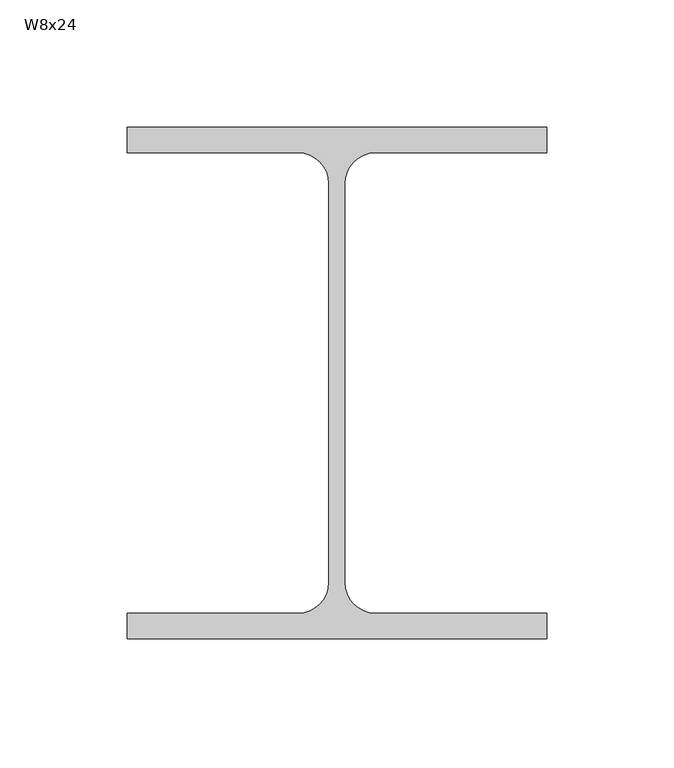
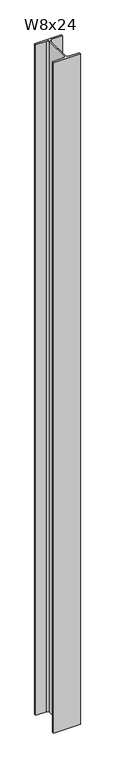
"""IFC4 building model written with IfcOpenShell, lengths in millimetres: column geometry, RME WF - Column : W8x24."""

import ifcopenshell
import ifcopenshell.guid

model = None  # the IFC model being written
_history = None  # IfcOwnerHistory: only IFC2X3 demands one
_inside = {}  # id of a spatial element -> (the spatial element, [elements in it])
_under = {}  # id of a project, library or spatial element -> (it, [spatial elements below it])
_declared = {}  # id of a project -> (the project, [libraries it declares])
_typed = {}  # id of a type object -> (the type object, [elements of that type])
_made_of = {}  # id of a material, layer set ... -> (it, [elements and type objects made of it])


def new_model(schema):
    """Start an empty IFC model of exactly this schema.

    Asked for "IFC4X3", IfcOpenShell would pick the latest addendum, in which some entities
    have other attributes; the version numbers below select the first issue.
    IFC2X3 requires an IfcOwnerHistory on every rooted entity: one is made here for all.
    """
    global model, _history
    if schema == "IFC4X3":
        model = ifcopenshell.file(schema_version=(4, 3, 0, 0))
    else:
        model = ifcopenshell.file(schema=schema)
    _inside.clear()
    _under.clear()
    _declared.clear()
    _typed.clear()
    _made_of.clear()
    _history = None
    if model.schema == "IFC2X3":
        org = make("IfcOrganization", Name="unknown")
        user = make(
            "IfcPersonAndOrganization",
            ThePerson=make("IfcPerson", FamilyName="unknown"),
            TheOrganization=org,
        )
        app = make(
            "IfcApplication",
            ApplicationDeveloper=org,
            Version="unknown",
            ApplicationFullName="unknown",
            ApplicationIdentifier="unknown",
        )
        _history = make(
            "IfcOwnerHistory",
            OwningUser=user,
            OwningApplication=app,
            ChangeAction="ADDED",
            CreationDate=0,
        )
    return model


def make(cls, **values):
    """One entity of the class cls with the attributes given. An attribute that is None is left unset."""
    return model.create_entity(
        cls, **{name: value for name, value in values.items() if value is not None}
    )


def rooted(cls, **values):
    """An entity with a GlobalId (a new one), such as an element, a storey or a relation."""
    return make(cls, GlobalId=ifcopenshell.guid.new(), OwnerHistory=_history, **values)


def si_unit(unit_type, name, prefix=None):
    """IfcSIUnit, for example si_unit("LENGTHUNIT", "METRE", prefix="MILLI")."""
    return make("IfcSIUnit", UnitType=unit_type, Prefix=prefix, Name=name)


def assignment(units):
    """IfcUnitAssignment: the units of a project."""
    return None if units is None else make("IfcUnitAssignment", Units=units)


def point(xyz):
    """IfcCartesianPoint."""
    return None if xyz is None else make("IfcCartesianPoint", Coordinates=xyz)


def direction(xyz):
    """IfcDirection."""
    return None if xyz is None else make("IfcDirection", DirectionRatios=xyz)


def frame(location, z_axis=None, x_axis=None):
    """IfcAxis2Placement3D, a coordinate frame: its origin and axes. An axis left out is left unset."""
    return make(
        "IfcAxis2Placement3D",
        Location=point(location),
        Axis=direction(z_axis),
        RefDirection=direction(x_axis),
    )


def frame_2d(location, x_axis=None):
    """IfcAxis2Placement2D, a coordinate frame in the plane: its origin and x axis."""
    return make(
        "IfcAxis2Placement2D", Location=point(location), RefDirection=direction(x_axis)
    )


def origin():
    """The frame at (0, 0, 0) with its axes left unset."""
    return frame((0.0, 0.0, 0.0))


def place(relative_to, where):
    """IfcLocalPlacement: puts the frame where relative to a parent placement (None: the world)."""
    return make(
        "IfcLocalPlacement", PlacementRelTo=relative_to, RelativePlacement=where
    )


def context(
    kind, dimensions, precision=None, world=None, true_north=None, identifier=None
):
    """IfcGeometricRepresentationContext, for example the 3D "Model" context."""
    return make(
        "IfcGeometricRepresentationContext",
        ContextIdentifier=identifier,
        ContextType=kind,
        CoordinateSpaceDimension=dimensions,
        Precision=precision,
        WorldCoordinateSystem=world,
        TrueNorth=true_north,
    )


def project(units=None, contexts=None):
    """IfcProject with its units and contexts."""
    return rooted(
        "IfcProject",
        Name="project",
        RepresentationContexts=contexts,
        UnitsInContext=assignment(units),
    )


def spatial(cls, under=None, at=None, **own):
    """A site, building, storey or space (cls), placed at a placement, below another one or the project."""
    s = rooted(cls, ObjectPlacement=at, **own)
    if under is not None:
        _under.setdefault(under.id(), (under, []))[1].append(s)
    return s


def polyline(points):
    """IfcPolyline through the points."""
    return make("IfcPolyline", Points=[point(p) for p in points])


def circle_curve(where, radius):
    """IfcCircle in the frame where."""
    return make("IfcCircle", Position=where, Radius=radius)


def trimmed(basis, trim1, trim2, sense, master):
    """IfcTrimmedCurve: the piece of a basis curve between two trims."""
    return make(
        "IfcTrimmedCurve",
        BasisCurve=basis,
        Trim1=trim1,
        Trim2=trim2,
        SenseAgreement=sense,
        MasterRepresentation=master,
    )


def segment(curve, same_sense, transition):
    """IfcCompositeCurveSegment."""
    return make(
        "IfcCompositeCurveSegment",
        Transition=transition,
        SameSense=same_sense,
        ParentCurve=curve,
    )


def composite_curve(segments, self_intersect=None):
    """IfcCompositeCurve: segments joined end to end."""
    return make("IfcCompositeCurve", Segments=segments, SelfIntersect=self_intersect)


def outline(outer, holes=None, kind="AREA"):
    """IfcArbitraryClosedProfileDef: a profile drawn as a closed curve; with holes, ...WithVoids."""
    if holes is None:
        return make("IfcArbitraryClosedProfileDef", ProfileType=kind, OuterCurve=outer)
    return make(
        "IfcArbitraryProfileDefWithVoids",
        ProfileType=kind,
        OuterCurve=outer,
        InnerCurves=holes,
    )


def extrude(swept, where, along, depth):
    """IfcExtrudedAreaSolid: the profile swept, set in the frame where, extruded along a direction by depth."""
    return make(
        "IfcExtrudedAreaSolid",
        SweptArea=swept,
        Position=where,
        ExtrudedDirection=direction(along),
        Depth=depth,
    )


def shape(context_of_items, identifier, shape_type, items):
    """IfcShapeRepresentation: the items that make up one representation, for example the "Body"."""
    return make(
        "IfcShapeRepresentation",
        ContextOfItems=context_of_items,
        RepresentationIdentifier=identifier,
        RepresentationType=shape_type,
        Items=items,
    )


def source(mapping_origin, context_of_items, identifier, shape_type, items):
    """IfcRepresentationMap: a shape defined once, which mapped items show again and again."""
    return make(
        "IfcRepresentationMap",
        MappingOrigin=mapping_origin,
        MappedRepresentation=shape(context_of_items, identifier, shape_type, items),
    )


def transform(
    local_origin,
    x_axis=None,
    y_axis=None,
    z_axis=None,
    scale=None,
    scale2=None,
    scale3=None,
    uniform=True,
):
    """IfcCartesianTransformationOperator3D, or its non-uniform kind. x_axis, y_axis, z_axis: its Axis1, 2, 3."""
    if uniform:
        return make(
            "IfcCartesianTransformationOperator3D",
            Axis1=direction(x_axis),
            Axis2=direction(y_axis),
            LocalOrigin=point(local_origin),
            Scale=scale,
            Axis3=direction(z_axis),
        )
    return make(
        "IfcCartesianTransformationOperator3DnonUniform",
        Axis1=direction(x_axis),
        Axis2=direction(y_axis),
        LocalOrigin=point(local_origin),
        Scale=scale,
        Axis3=direction(z_axis),
        Scale2=scale2,
        Scale3=scale3,
    )


def mapped(mapping_source, mapping_target):
    """IfcMappedItem: shows the shape of a source again, moved by a transform."""
    return make(
        "IfcMappedItem", MappingSource=mapping_source, MappingTarget=mapping_target
    )


def made_of(thing, what):
    """Note that an element or type object is made of a material, layer set ...; save() writes the relation."""
    if what is not None:
        _made_of.setdefault(what.id(), (what, []))[1].append(thing)
    return thing


def element(
    cls,
    number,
    at=None,
    inside=None,
    cuts=None,
    type_object=None,
    material=None,
    context=None,
    identifier="Body",
    shape_type=None,
    held_by="IfcProductDefinitionShape",
    body=None,
    shapes=None,
    **own,
):
    """One element of the class cls, such as IfcWall. Its Tag is "e" and its number.

    at: its placement. inside: the storey or other place that contains it. cuts: it is an
    opening in that element (IfcRelVoidsElement). A single representation is given by context,
    identifier, shape_type and body (its items); several are given by shapes. held_by: the class
    of the entity that holds the representations. save() writes the other relations.
    """
    e = rooted(cls, Tag="e%d" % number, ObjectPlacement=at, **own)
    if body is not None:
        shapes = [shape(context, identifier, shape_type, body)]
    if shapes is not None:
        e.Representation = make(held_by, Representations=shapes)
    if inside is not None:
        _inside.setdefault(inside.id(), (inside, []))[1].append(e)
    if cuts is not None:
        rooted(
            "IfcRelVoidsElement", RelatingBuildingElement=cuts, RelatedOpeningElement=e
        )
    if type_object is not None:
        _typed.setdefault(type_object.id(), (type_object, []))[1].append(e)
    return made_of(e, material)


def aggregate(whole, parts):
    """IfcRelAggregates: a whole, such as a stair, and the parts it consists of."""
    return rooted("IfcRelAggregates", RelatingObject=whole, RelatedObjects=parts)


def save(model, path):
    """Write the relations noted so far, then the file.

    IfcRelAggregates (storeys below a building ...), IfcRelContainedInSpatialStructure (elements
    in a storey), IfcRelDefinesByType, IfcRelAssociatesMaterial and IfcRelDeclares: one each for
    every whole, place, type object, material and project.
    """
    for whole, parts in _under.values():
        aggregate(whole, parts)
    for where, things in _inside.values():
        rooted(
            "IfcRelContainedInSpatialStructure",
            RelatedElements=things,
            RelatingStructure=where,
        )
    for kind, things in _typed.values():
        rooted("IfcRelDefinesByType", RelatedObjects=things, RelatingType=kind)
    for what, things in _made_of.values():
        rooted("IfcRelAssociatesMaterial", RelatedObjects=things, RelatingMaterial=what)
    for by, libraries in _declared.values():
        rooted("IfcRelDeclares", RelatingContext=by, RelatedDefinitions=libraries)
    model.write(path)


def w8x24_4b7dde36(model_context):
    return source(origin(), model_context, "Body", "SweptSolid", [
        extrude(outline(composite_curve([segment(polyline([(82.55, 100.711), (82.55, 90.551), (15.1765, 90.551)]), True, "CONTINUOUS"), segment(trimmed(circle_curve(frame_2d((15.1765, 78.486)), 12.065), [point((15.1765, 90.551))], [point((3.1115, 78.486))], True, "CARTESIAN"), True, "CONTINUOUS"), segment(polyline([(3.1115, 78.486), (3.1115, -78.486)]), True, "CONTINUOUS"), segment(trimmed(circle_curve(frame_2d((15.1765, -78.486)), 12.065), [point((3.1115, -78.486))], [point((15.1765, -90.551))], True, "CARTESIAN"), True, "CONTINUOUS"), segment(polyline([(15.1765, -90.551), (82.55, -90.551), (82.55, -100.711), (-82.55, -100.711), (-82.55, -90.551), (-15.1765, -90.551)]), True, "CONTINUOUS"), segment(trimmed(circle_curve(frame_2d((-15.1765, -78.486)), 12.065), [point((-15.1765, -90.551))], [point((-3.1115, -78.486))], True, "CARTESIAN"), True, "CONTINUOUS"), segment(polyline([(-3.1115, -78.486), (-3.1115, 78.486)]), True, "CONTINUOUS"), segment(trimmed(circle_curve(frame_2d((-15.1765, 78.486)), 12.065), [point((-3.1115, 78.486))], [point((-15.1765, 90.551))], True, "CARTESIAN"), True, "CONTINUOUS"), segment(polyline([(-15.1765, 90.551), (-82.55, 90.551), (-82.55, 100.711), (82.55, 100.711)]), True, "CONTINUOUS")], self_intersect=False)), frame((0.0, 0.0, -304.8), z_axis=(0.0, 0.0, 1.0), x_axis=(1.0, 0.0, 0.0)), (0.0, 0.0, 1.0), 4368.8),
    ])


if __name__ == "__main__":
    model = new_model("IFC4")
    model_context = context("Model", 3, world=origin())
    ifc_project = project(units=[si_unit("LENGTHUNIT", "METRE", prefix="MILLI")], contexts=[model_context])
    site = spatial("IfcSite", under=ifc_project)
    building = spatial("IfcBuilding", under=site)
    placement = place(None, origin())
    w8x24_shape = w8x24_4b7dde36(model_context)
    element("IfcColumn", 1, ObjectType="RME WF - Column : W8x24", at=placement, inside=building, context=model_context, shape_type="MappedRepresentation", body=[
        mapped(w8x24_shape, transform((0.0, 0.0, 0.0), x_axis=(1.0, 0.0, 0.0), y_axis=(0.0, 1.0, 0.0), z_axis=(0.0, 0.0, 1.0))),
    ])
    save(model, "model.ifc")

# Revit data of these elements
# Type "RME WF - Column : W8x24"
#   Type Mark = "C1"
#   REINF TYPE [instance default] = ""
#   Nominal Size = "W16"
#   COL REMARKS [instance default] = ""
#   BP [instance default] = ""
#   Assembly Code = "B10"
#   W = 24
#   bf = 0' - 6 1/2"
#   d = 0' - 7.93"
#   k = 0' - 0 7/8"
#   kr = 0' - 0.475"
#   tf = 0' - 0.4"
#   tw = 0' - 0.245"
#   A = 0.0491667 SF
#   Structural Material [instance default] = Metal - Steel - ASTM A992
# Element 1 (IfcColumn, "RME WF - Column : W8x24")
#   Materials on its faces: "Metal - Steel - ASTM A992"
# Materials
#   "Metal - Steel - ASTM A992": class "Metal", colour RGB 255 128 0, transparency 0
